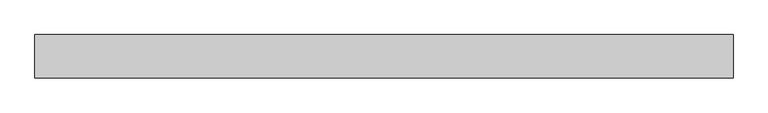
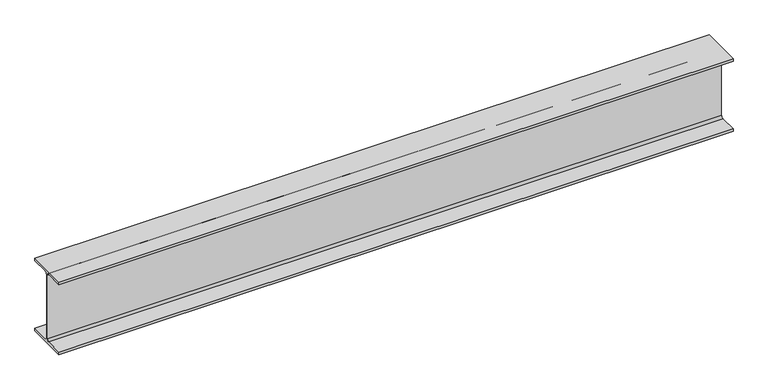
"""IFC4 building model written with IfcOpenShell, lengths in millimetres: beam geometry, Old_Steel Beam_H-KSD3502 : H_SB_ASB_H-200×200x8x12."""

from ifc_helpers import new_model, si_unit, point, frame, frame_2d, origin, place, context, project, spatial, polyline, circle_curve, trimmed, segment, composite_curve, outline, extrude, source, transform, mapped, element, save


def beam_d1301045(model_context):
    return source(origin(), model_context, "Body", "SweptSolid", [
        extrude(outline(composite_curve([segment(polyline([(82.5, -141.5), (82.5, -151.7), (-82.5, -151.7), (-82.5, -141.5), (-11.9, -141.5)]), True, "CONTINUOUS"), segment(trimmed(circle_curve(frame_2d((-11.9, -132.6)), 8.9), [point((-11.9, -141.5))], [point((-3.0, -132.6))], True, "CARTESIAN"), True, "CONTINUOUS"), segment(polyline([(-3.0, -132.6), (-3.0, 132.6)]), True, "CONTINUOUS"), segment(trimmed(circle_curve(frame_2d((-11.9, 132.6)), 8.9), [point((-3.0, 132.6))], [point((-11.9, 141.5))], True, "CARTESIAN"), True, "CONTINUOUS"), segment(polyline([(-11.9, 141.5), (-82.5, 141.5), (-82.5, 151.7), (82.5, 151.7), (82.5, 141.5), (11.9, 141.5)]), True, "CONTINUOUS"), segment(trimmed(circle_curve(frame_2d((11.9, 132.6)), 8.9), [point((11.9, 141.5))], [point((3.0, 132.6))], True, "CARTESIAN"), True, "CONTINUOUS"), segment(polyline([(3.0, 132.6), (3.0, -132.6)]), True, "CONTINUOUS"), segment(trimmed(circle_curve(frame_2d((11.9, -132.6)), 8.9), [point((3.0, -132.6))], [point((11.9, -141.5))], True, "CARTESIAN"), True, "CONTINUOUS"), segment(polyline([(11.9, -141.5), (82.5, -141.5)]), True, "CONTINUOUS")], self_intersect=False)), frame((-1341.7710002, 0.0, 0.0), z_axis=(1.0, 0.0, 0.0), x_axis=(0.0, 1.0, 0.0)), (0.0, 0.0, 1.0), 2665.7394563),
    ])


if __name__ == "__main__":
    model = new_model("IFC4")
    model_context = context("Model", 3, world=origin())
    ifc_project = project(units=[si_unit("LENGTHUNIT", "METRE", prefix="MILLI")], contexts=[model_context])
    site = spatial("IfcSite", under=ifc_project)
    building = spatial("IfcBuilding", under=site)
    placement = place(None, origin())
    beam_shape = beam_d1301045(model_context)
    element("IfcBeam", 1, ObjectType="Old_Steel Beam_H-KSD3502 : H_SB_ASB_H-200×200x8x12", at=placement, inside=building, context=model_context, shape_type="MappedRepresentation", body=[
        mapped(beam_shape, transform((0.0, 0.0, 0.0), x_axis=(1.0, 0.0, 0.0), y_axis=(0.0, 1.0, 0.0), z_axis=(0.0, 0.0, 1.0))),
    ])
    save(model, "model.ifc")

# Revit data of these elements
# Type "Old_Steel Beam_H-KSD3502 : H_SB_ASB_H-200×200x8x12"
#   Width = 20.0 cm
#   Web Thickness = 0.8 cm
#   Web Fillet = 1.3 cm
#   Warping Constant = 141376.0 cm⁶
#   Torsional Moment of Inertia = 26.2485 cm⁴
#   Torsional Modulus = 1.0 cm³
#   Section Area = 63.53 cm²
#   Plastic Modulus weak axis = 244.0 cm³
#   Plastic Modulus strong axis = 525.0 cm³
#   Perimeter = 1.16 m²/m
#   Nominal Weight = 49.90 kgf/m
#   Moment of Inertia weak axis = 1600.00 cm⁴
#   Moment of Inertia strong axis = 4720.00 cm⁴
#   Height = 20.0 cm
#   Flange Thickness = 1.2 cm
#   Elastic Modulus weak axis = 160.0 cm³
#   Elastic Modulus strong axis = 472.0 cm³
#   Centroid Vertical = 10.0 cm
#   Centroid Horizontal = 10.0 cm
#   Length [instance default] = 1.5240 m
#   Structural Material [instance default] = Steel, 45-345
#   Assembly Code = ""
# Element 1 (IfcBeam, "Old_Steel Beam_H-KSD3502 : H_SB_ASB_H-200×200x8x12")
#   Structural Material = none
# Materials
#   "Steel, 45-345": class "Metal", colour RGB 189 187 185, transparency 0, Description = "Steel 345 MPa", Cost = 0
